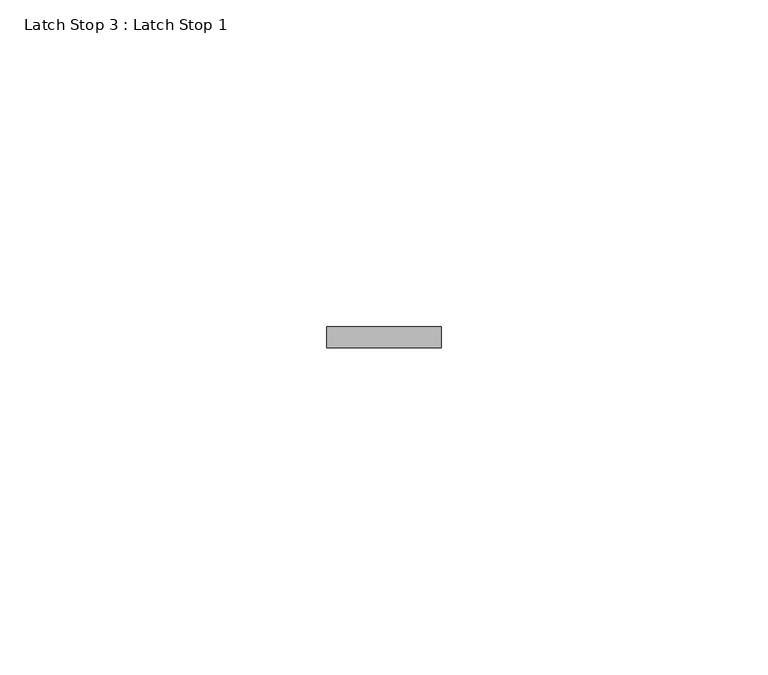
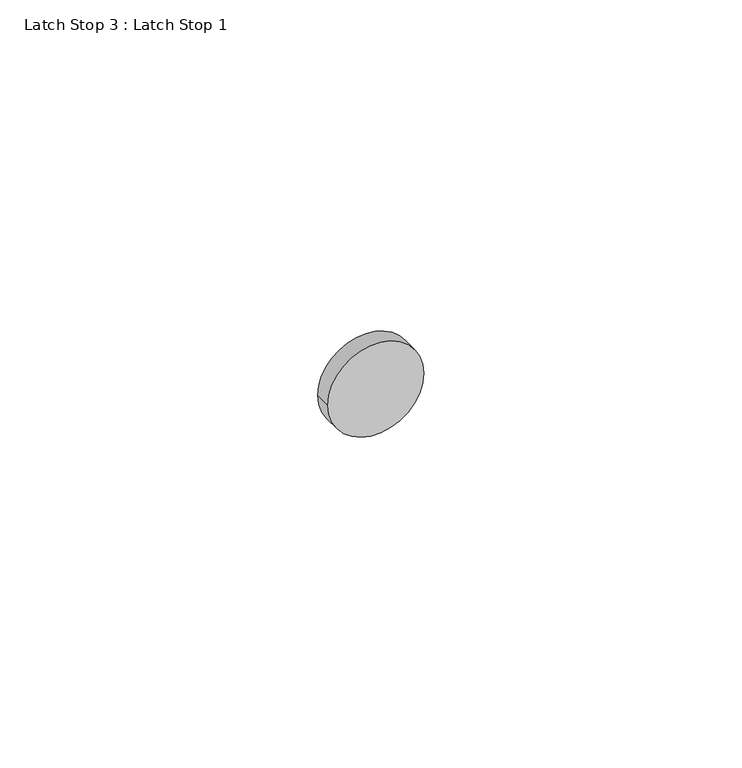
"""IFC4 building model written with IfcOpenShell, lengths in millimetres: proxy geometry, Latch Stop 3 : Latch Stop 1."""

from ifc_helpers import new_model, si_unit, point, frame, frame_2d, origin, place, context, project, spatial, circle_curve, trimmed, segment, composite_curve, outline, extrude, source, transform, mapped, element, save


def latch_stop_3_latch_stop_1_4e8d7d1d(model_context):
    return source(origin(), model_context, "Body", "SweptSolid", [
        extrude(outline(composite_curve([segment(trimmed(circle_curve(frame_2d((1066.8, 587312.7185739)), 8.73125), [point((1066.8, 587303.9873239))], [point((1066.8, 587321.4498239))], False, "CARTESIAN"), True, "CONTINUOUS"), segment(trimmed(circle_curve(frame_2d((1066.8, 587312.7185739)), 8.73125), [point((1066.8, 587321.4498239))], [point((1066.8, 587303.9873239))], False, "CARTESIAN"), True, "CONTINUOUS")], self_intersect=False)), frame((0.0, -535166.6413841, 0.0), z_axis=(0.0, 1.0, 0.0), x_axis=(0.0, 0.0, 1.0)), (0.0, 0.0, 1.0), 3.175),
    ])


if __name__ == "__main__":
    model = new_model("IFC4")
    model_context = context("Model", 3, world=origin())
    ifc_project = project(units=[si_unit("LENGTHUNIT", "METRE", prefix="MILLI")], contexts=[model_context])
    site = spatial("IfcSite", under=ifc_project)
    building = spatial("IfcBuilding", under=site)
    placement = place(None, origin())
    latch_stop_3_latch_stop_1_shape = latch_stop_3_latch_stop_1_4e8d7d1d(model_context)
    element("IfcBuildingElementProxy", 1, Name="Latch Stop 3 : Latch Stop 1", ObjectType="Latch Stop 3 : Latch Stop 1", at=placement, inside=building, context=model_context, shape_type="MappedRepresentation", body=[
        mapped(latch_stop_3_latch_stop_1_shape, transform((0.0, 0.0, 0.0), x_axis=(1.0, 0.0, 0.0), y_axis=(0.0, 1.0, 0.0), z_axis=(0.0, 0.0, 1.0))),
    ])
    save(model, "model.ifc")

# Revit data of these elements
# Element 1 (IfcBuildingElementProxy, "Latch Stop 3 : Latch Stop 1")
#   Materials on its faces: "GALV. GATE LATCH"
# Materials
#   "GALV. GATE LATCH": class "Metal", colour RGB 189 187 185, transparency 0, Description = "Carbon steel", Cost = 0
